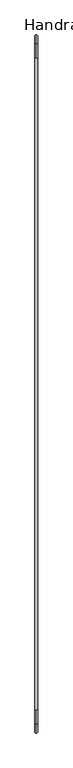
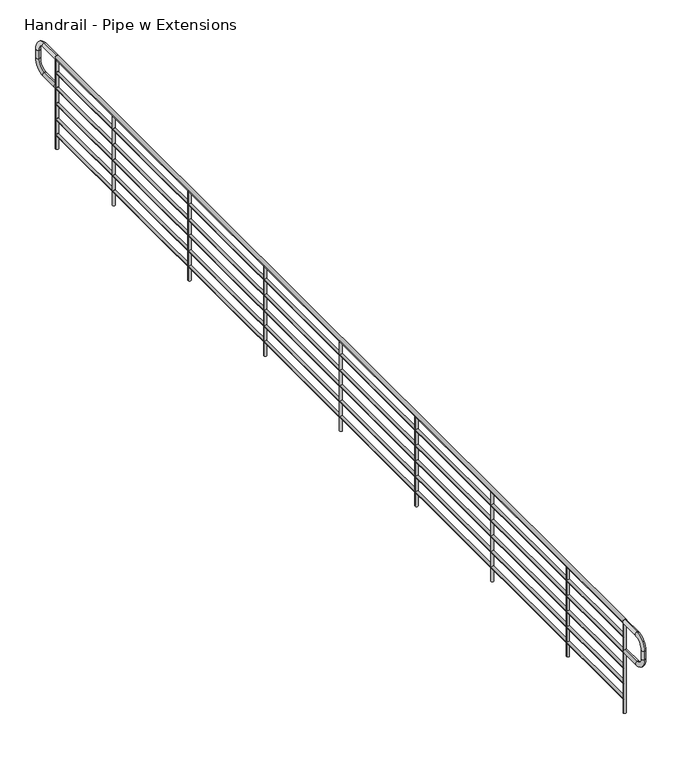
"""IFC4 building model written with IfcOpenShell, lengths in millimetres: railing geometry, Handrail - Pipe w Extensions."""

from ifc_helpers import new_model, si_unit, point, frame, frame_2d, origin, origin_with_axes, place, context, project, spatial, circle_curve, ellipse_curve, trimmed, segment, composite_curve, outline, extrude, source, transform, mapped, element, save
from ifc_brep_helpers import plane_surface, cylinder_surface, revolved_surface, advanced_brep


def handrail_pipe_w_extensions_4fdb8f92(model_context):
    return source(origin(), model_context, "Body", "SolidModel", [
        extrude(outline(composite_curve([segment(trimmed(circle_curve(frame_2d((895.35, -1497.5978678)), 19.05), [point((895.35, -1478.5478678))], [point((895.35, -1516.6478678))], False, "CARTESIAN"), True, "CONTINUOUS"), segment(trimmed(circle_curve(frame_2d((895.35, -1497.5978678)), 19.05), [point((895.35, -1516.6478678))], [point((895.35, -1478.5478678))], False, "CARTESIAN"), True, "CONTINUOUS")], self_intersect=False)), frame((0.0, -14489.4143828, 0.0), z_axis=(0.0, 1.0, 0.0), x_axis=(0.0, 0.0, 1.0)), (0.0, 0.0, 1.0), 9144.0),
        extrude(outline(composite_curve([segment(trimmed(circle_curve(frame_2d((749.3, -1497.5978678)), 12.7), [point((749.3, -1484.8978678))], [point((749.3, -1510.2978678))], False, "CARTESIAN"), True, "CONTINUOUS"), segment(trimmed(circle_curve(frame_2d((749.3, -1497.5978678)), 12.7), [point((749.3, -1510.2978678))], [point((749.3, -1484.8978678))], False, "CARTESIAN"), True, "CONTINUOUS")], self_intersect=False)), frame((0.0, -14489.4143828, 0.0), z_axis=(0.0, 1.0, 0.0), x_axis=(0.0, 0.0, 1.0)), (0.0, 0.0, 1.0), 9144.0),
        extrude(outline(composite_curve([segment(trimmed(circle_curve(frame_2d((596.9, -1497.5978678)), 12.7), [point((596.9, -1484.8978678))], [point((596.9, -1510.2978678))], False, "CARTESIAN"), True, "CONTINUOUS"), segment(trimmed(circle_curve(frame_2d((596.9, -1497.5978678)), 12.7), [point((596.9, -1510.2978678))], [point((596.9, -1484.8978678))], False, "CARTESIAN"), True, "CONTINUOUS")], self_intersect=False)), frame((0.0, -14489.4143828, 0.0), z_axis=(0.0, 1.0, 0.0), x_axis=(0.0, 0.0, 1.0)), (0.0, 0.0, 1.0), 9144.0),
        extrude(outline(composite_curve([segment(trimmed(circle_curve(frame_2d((444.5, -1497.5978678)), 12.7), [point((444.5, -1484.8978678))], [point((444.5, -1510.2978678))], False, "CARTESIAN"), True, "CONTINUOUS"), segment(trimmed(circle_curve(frame_2d((444.5, -1497.5978678)), 12.7), [point((444.5, -1510.2978678))], [point((444.5, -1484.8978678))], False, "CARTESIAN"), True, "CONTINUOUS")], self_intersect=False)), frame((0.0, -14489.4143828, 0.0), z_axis=(0.0, 1.0, 0.0), x_axis=(0.0, 0.0, 1.0)), (0.0, 0.0, 1.0), 9144.0),
        extrude(outline(composite_curve([segment(trimmed(circle_curve(frame_2d((292.1, -1497.5978678)), 12.7), [point((292.1, -1484.8978678))], [point((292.1, -1510.2978678))], False, "CARTESIAN"), True, "CONTINUOUS"), segment(trimmed(circle_curve(frame_2d((292.1, -1497.5978678)), 12.7), [point((292.1, -1510.2978678))], [point((292.1, -1484.8978678))], False, "CARTESIAN"), True, "CONTINUOUS")], self_intersect=False)), frame((0.0, -14489.4143828, 0.0), z_axis=(0.0, 1.0, 0.0), x_axis=(0.0, 0.0, 1.0)), (0.0, 0.0, 1.0), 9144.0),
        extrude(outline(composite_curve([segment(trimmed(circle_curve(frame_2d((139.7, -1497.5978678)), 12.7), [point((139.7, -1484.8978678))], [point((139.7, -1510.2978678))], False, "CARTESIAN"), True, "CONTINUOUS"), segment(trimmed(circle_curve(frame_2d((139.7, -1497.5978678)), 12.7), [point((139.7, -1510.2978678))], [point((139.7, -1484.8978678))], False, "CARTESIAN"), True, "CONTINUOUS")], self_intersect=False)), frame((0.0, -14489.4143828, 0.0), z_axis=(0.0, 1.0, 0.0), x_axis=(0.0, 0.0, 1.0)), (0.0, 0.0, 1.0), 9144.0),
        extrude(outline(composite_curve([segment(trimmed(circle_curve(frame_2d((-1497.5978678, -13575.0143828)), 12.7), [point((-1484.8978678, -13575.0143828))], [point((-1510.2978678, -13575.0143828))], False, "CARTESIAN"), True, "CONTINUOUS"), segment(trimmed(circle_curve(frame_2d((-1497.5978678, -13575.0143828)), 12.7), [point((-1510.2978678, -13575.0143828))], [point((-1484.8978678, -13575.0143828))], False, "CARTESIAN"), True, "CONTINUOUS")], self_intersect=False)), origin_with_axes(), (0.0, 0.0, 1.0), 876.3),
        extrude(outline(composite_curve([segment(trimmed(circle_curve(frame_2d((-1497.5978678, -12355.8143828)), 12.7), [point((-1484.8978678, -12355.8143828))], [point((-1510.2978678, -12355.8143828))], False, "CARTESIAN"), True, "CONTINUOUS"), segment(trimmed(circle_curve(frame_2d((-1497.5978678, -12355.8143828)), 12.7), [point((-1510.2978678, -12355.8143828))], [point((-1484.8978678, -12355.8143828))], False, "CARTESIAN"), True, "CONTINUOUS")], self_intersect=False)), origin_with_axes(), (0.0, 0.0, 1.0), 876.3),
        extrude(outline(composite_curve([segment(trimmed(circle_curve(frame_2d((-1497.5978678, -11136.6143828)), 12.7), [point((-1484.8978678, -11136.6143828))], [point((-1510.2978678, -11136.6143828))], False, "CARTESIAN"), True, "CONTINUOUS"), segment(trimmed(circle_curve(frame_2d((-1497.5978678, -11136.6143828)), 12.7), [point((-1510.2978678, -11136.6143828))], [point((-1484.8978678, -11136.6143828))], False, "CARTESIAN"), True, "CONTINUOUS")], self_intersect=False)), origin_with_axes(), (0.0, 0.0, 1.0), 876.3),
        extrude(outline(composite_curve([segment(trimmed(circle_curve(frame_2d((-1497.5978678, -9917.4143828)), 12.7), [point((-1484.8978678, -9917.4143828))], [point((-1510.2978678, -9917.4143828))], False, "CARTESIAN"), True, "CONTINUOUS"), segment(trimmed(circle_curve(frame_2d((-1497.5978678, -9917.4143828)), 12.7), [point((-1510.2978678, -9917.4143828))], [point((-1484.8978678, -9917.4143828))], False, "CARTESIAN"), True, "CONTINUOUS")], self_intersect=False)), origin_with_axes(), (0.0, 0.0, 1.0), 876.3),
        extrude(outline(composite_curve([segment(trimmed(circle_curve(frame_2d((-1497.5978678, -8698.2143828)), 12.7), [point((-1484.8978678, -8698.2143828))], [point((-1510.2978678, -8698.2143828))], False, "CARTESIAN"), True, "CONTINUOUS"), segment(trimmed(circle_curve(frame_2d((-1497.5978678, -8698.2143828)), 12.7), [point((-1510.2978678, -8698.2143828))], [point((-1484.8978678, -8698.2143828))], False, "CARTESIAN"), True, "CONTINUOUS")], self_intersect=False)), origin_with_axes(), (0.0, 0.0, 1.0), 876.3),
        extrude(outline(composite_curve([segment(trimmed(circle_curve(frame_2d((-1497.5978678, -7479.0143828)), 12.7), [point((-1484.8978678, -7479.0143828))], [point((-1510.2978678, -7479.0143828))], False, "CARTESIAN"), True, "CONTINUOUS"), segment(trimmed(circle_curve(frame_2d((-1497.5978678, -7479.0143828)), 12.7), [point((-1510.2978678, -7479.0143828))], [point((-1484.8978678, -7479.0143828))], False, "CARTESIAN"), True, "CONTINUOUS")], self_intersect=False)), origin_with_axes(), (0.0, 0.0, 1.0), 876.3),
        extrude(outline(composite_curve([segment(trimmed(circle_curve(frame_2d((-1497.5978678, -6259.8143828)), 12.7), [point((-1484.8978678, -6259.8143828))], [point((-1510.2978678, -6259.8143828))], False, "CARTESIAN"), True, "CONTINUOUS"), segment(trimmed(circle_curve(frame_2d((-1497.5978678, -6259.8143828)), 12.7), [point((-1510.2978678, -6259.8143828))], [point((-1484.8978678, -6259.8143828))], False, "CARTESIAN"), True, "CONTINUOUS")], self_intersect=False)), origin_with_axes(), (0.0, 0.0, 1.0), 876.3),
        advanced_brep(
        [(-1497.5978678, -14502.1143828, 628.65), (-1497.5978678, -14502.1143828, 590.55), (-1497.5978678, -14692.6143828, 628.65), (-1497.5978678, -14692.6143828, 590.55), (-1497.5978678, -14813.2643828, 711.2), (-1497.5978678, -14775.1643828, 711.2), (-1497.5978678, -14775.1643828, 793.75), (-1497.5978678, -14813.2643828, 793.75), (-1497.5978678, -14692.6143828, 914.4), (-1497.5978678, -14692.6143828, 876.3), (-1497.5978678, -14489.4143828, 876.3), (-1497.5978678, -14489.4143828, 914.4)],
        [
            (0, 1, circle_curve(frame((-1497.5978678, -14502.1143828, 609.6), z_axis=(0.0, 1.0, 0.0), x_axis=(0.0, 0.0, -1.0)), 19.05)),
            (1, 0, circle_curve(frame((-1497.5978678, -14502.1143828, 609.6), z_axis=(0.0, 1.0, 0.0), x_axis=(0.0, 0.0, -1.0)), 19.05)),
            (0, 2),
            (2, 3, circle_curve(frame((-1497.5978678, -14692.6143828, 609.6), z_axis=(0.0, 1.0, 0.0), x_axis=(0.0, 0.0, -1.0)), 19.05)),
            (3, 1),
            (3, 2, circle_curve(frame((-1497.5978678, -14692.6143828, 609.6), z_axis=(0.0, 1.0, 0.0), x_axis=(0.0, 0.0, -1.0)), 19.05)),
            (4, 3, circle_curve(frame((-1497.5978678, -14692.6143828, 711.2), z_axis=(1.0, 0.0, 0.0), x_axis=(0.0, 0.0, -1.0)), 120.65)),
            (2, 5, circle_curve(frame((-1497.5978678, -14692.6143828, 711.2), z_axis=(-1.0, 0.0, 0.0), x_axis=(0.0, 0.0, -1.0)), 82.55)),
            (5, 4, circle_curve(frame((-1497.5978678, -14794.2143828, 711.2), z_axis=(0.0, 0.0, -1.0), x_axis=(0.0, -1.0, 0.0)), 19.05)),
            (4, 5, circle_curve(frame((-1497.5978678, -14794.2143828, 711.2), z_axis=(0.0, 0.0, -1.0), x_axis=(0.0, -1.0, 0.0)), 19.05)),
            (5, 6),
            (6, 7, circle_curve(frame((-1497.5978678, -14794.2143828, 793.75), z_axis=(0.0, 0.0, -1.0), x_axis=(0.0, -1.0, 0.0)), 19.05)),
            (7, 4),
            (7, 6, circle_curve(frame((-1497.5978678, -14794.2143828, 793.75), z_axis=(0.0, 0.0, -1.0), x_axis=(0.0, -1.0, 0.0)), 19.05)),
            (8, 7, circle_curve(frame((-1497.5978678, -14692.6143828, 793.75), z_axis=(1.0, 0.0, 0.0), x_axis=(0.0, -1.0, 0.0)), 120.65)),
            (6, 9, circle_curve(frame((-1497.5978678, -14692.6143828, 793.75), z_axis=(-1.0, 0.0, 0.0), x_axis=(0.0, -1.0, 0.0)), 82.55)),
            (9, 8, circle_curve(frame((-1497.5978678, -14692.6143828, 895.35), z_axis=(0.0, -1.0, 0.0), x_axis=(0.0, 0.0, 1.0)), 19.05)),
            (8, 9, circle_curve(frame((-1497.5978678, -14692.6143828, 895.35), z_axis=(0.0, -1.0, 0.0), x_axis=(0.0, 0.0, 1.0)), 19.05)),
            (10, 11, circle_curve(frame((-1497.5978678, -14489.4143828, 895.35), z_axis=(0.0, 1.0, 0.0), x_axis=(0.0, 0.0, 1.0)), 19.05)),
            (11, 10, circle_curve(frame((-1497.5978678, -14489.4143828, 895.35), z_axis=(0.0, 1.0, 0.0), x_axis=(0.0, 0.0, 1.0)), 19.05)),
            (9, 10),
            (11, 8),
        ],
        [
            plane_surface(frame((-1516.6478678, -14502.1143828, 609.6), z_axis=(0.0, 1.0, 0.0), x_axis=(0.0, 0.0, -1.0))),
            cylinder_surface(frame((-1497.5978678, -14502.1143828, 609.6), z_axis=(0.0, 1.0, 0.0), x_axis=(0.0, 0.0, -1.0)), 19.05),
            revolved_surface(trimmed(ellipse_curve(frame((-1497.5978678, -14692.6143828, 609.6), z_axis=(0.0, 1.0, 0.0), x_axis=(0.0, 0.0, -1.0)), 19.05, 19.05), [point((-1497.5978678, -14692.6143828, 628.65))], [point((-1497.5978678, -14692.6143828, 590.55))], True, "CARTESIAN"), (-1497.5978678, -14692.6143828, 711.2), (-1.0, 0.0, 0.0)),
            revolved_surface(trimmed(ellipse_curve(frame((-1497.5978678, -14692.6143828, 609.6), z_axis=(0.0, 1.0, 0.0), x_axis=(0.0, 0.0, -1.0)), 19.05, 19.05), [point((-1497.5978678, -14692.6143828, 590.55))], [point((-1497.5978678, -14692.6143828, 628.65))], True, "CARTESIAN"), (-1497.5978678, -14692.6143828, 711.2), (-1.0, 0.0, 0.0)),
            cylinder_surface(frame((-1497.5978678, -14794.2143828, 711.2), z_axis=(0.0, 0.0, -1.0), x_axis=(0.0, -1.0, 0.0)), 19.05),
            revolved_surface(trimmed(ellipse_curve(frame((-1497.5978678, -14794.2143828, 793.75), z_axis=(0.0, 0.0, -1.0), x_axis=(0.0, -1.0, 0.0)), 19.05, 19.05), [point((-1497.5978678, -14775.1643828, 793.75))], [point((-1497.5978678, -14813.2643828, 793.75))], True, "CARTESIAN"), (-1497.5978678, -14692.6143828, 793.75), (-1.0, 0.0, 0.0)),
            revolved_surface(trimmed(ellipse_curve(frame((-1497.5978678, -14794.2143828, 793.75), z_axis=(0.0, 0.0, -1.0), x_axis=(0.0, -1.0, 0.0)), 19.05, 19.05), [point((-1497.5978678, -14813.2643828, 793.75))], [point((-1497.5978678, -14775.1643828, 793.75))], True, "CARTESIAN"), (-1497.5978678, -14692.6143828, 793.75), (-1.0, 0.0, 0.0)),
            plane_surface(frame((-1516.6478678, -14489.4143828, 895.35), z_axis=(0.0, 1.0, 0.0), x_axis=(0.0, 0.0, 1.0))),
            cylinder_surface(frame((-1497.5978678, -14692.6143828, 895.35), z_axis=(0.0, -1.0, 0.0), x_axis=(0.0, 0.0, 1.0)), 19.05),
        ],
        [
            (0, [[1, 2]]),
            (1, [[-1, 3, 4, 5]]),
            (1, [[-2, -5, 6, -3]]),
            (2, [[7, -4, 8, 9]]),
            (3, [[-8, -6, -7, 10]]),
            (4, [[-9, 11, 12, 13]]),
            (4, [[-10, -13, 14, -11]]),
            (5, [[15, -12, 16, 17]]),
            (6, [[-16, -14, -15, 18]]),
            (7, [[19, 20]]),
            (8, [[-17, 21, -20, 22]]),
            (8, [[-18, -22, -19, -21]]),
        ],
    ),
        extrude(outline(composite_curve([segment(trimmed(circle_curve(frame_2d((-1497.5978678, -14489.4143828)), 12.7), [point((-1510.2978678, -14489.4143828))], [point((-1484.8978678, -14489.4143828))], False, "CARTESIAN"), True, "CONTINUOUS"), segment(trimmed(circle_curve(frame_2d((-1497.5978678, -14489.4143828)), 12.7), [point((-1484.8978678, -14489.4143828))], [point((-1510.2978678, -14489.4143828))], False, "CARTESIAN"), True, "CONTINUOUS")], self_intersect=False)), origin_with_axes(), (0.0, 0.0, 1.0), 876.3),
        advanced_brep(
        [(-1497.5978678, -5345.4143828, 876.3), (-1497.5978678, -5345.4143828, 914.4), (-1497.5978678, -5142.2143828, 876.3), (-1497.5978678, -5142.2143828, 914.4), (-1497.5978678, -5021.5643828, 793.75), (-1497.5978678, -5059.6643828, 793.75), (-1497.5978678, -5059.6643828, 711.2), (-1497.5978678, -5021.5643828, 711.2), (-1497.5978678, -5142.2143828, 590.55), (-1497.5978678, -5142.2143828, 628.65), (-1497.5978678, -5332.7143828, 628.65), (-1497.5978678, -5332.7143828, 590.55)],
        [
            (0, 1, circle_curve(frame((-1497.5978678, -5345.4143828, 895.35), z_axis=(0.0, -1.0, 0.0), x_axis=(0.0, 0.0, 1.0)), 19.05)),
            (1, 0, circle_curve(frame((-1497.5978678, -5345.4143828, 895.35), z_axis=(0.0, -1.0, 0.0), x_axis=(0.0, 0.0, 1.0)), 19.05)),
            (0, 2),
            (2, 3, circle_curve(frame((-1497.5978678, -5142.2143828, 895.35), z_axis=(0.0, -1.0, 0.0), x_axis=(0.0, 0.0, 1.0)), 19.05)),
            (3, 1),
            (3, 2, circle_curve(frame((-1497.5978678, -5142.2143828, 895.35), z_axis=(0.0, -1.0, 0.0), x_axis=(0.0, 0.0, 1.0)), 19.05)),
            (4, 3, circle_curve(frame((-1497.5978678, -5142.2143828, 793.75), z_axis=(1.0, 0.0, 0.0), x_axis=(0.0, 0.0, 1.0)), 120.65)),
            (2, 5, circle_curve(frame((-1497.5978678, -5142.2143828, 793.75), z_axis=(-1.0, 0.0, 0.0), x_axis=(0.0, 0.0, 1.0)), 82.55)),
            (5, 4, circle_curve(frame((-1497.5978678, -5040.6143828, 793.75), z_axis=(0.0, 0.0, 1.0), x_axis=(0.0, 1.0, 0.0)), 19.05)),
            (4, 5, circle_curve(frame((-1497.5978678, -5040.6143828, 793.75), z_axis=(0.0, 0.0, 1.0), x_axis=(0.0, 1.0, 0.0)), 19.05)),
            (5, 6),
            (6, 7, circle_curve(frame((-1497.5978678, -5040.6143828, 711.2), z_axis=(0.0, 0.0, 1.0), x_axis=(0.0, 1.0, 0.0)), 19.05)),
            (7, 4),
            (7, 6, circle_curve(frame((-1497.5978678, -5040.6143828, 711.2), z_axis=(0.0, 0.0, 1.0), x_axis=(0.0, 1.0, 0.0)), 19.05)),
            (8, 7, circle_curve(frame((-1497.5978678, -5142.2143828, 711.2), z_axis=(1.0, 0.0, 0.0), x_axis=(0.0, 1.0, 0.0)), 120.65)),
            (6, 9, circle_curve(frame((-1497.5978678, -5142.2143828, 711.2), z_axis=(-1.0, 0.0, 0.0), x_axis=(0.0, 1.0, 0.0)), 82.55)),
            (9, 8, circle_curve(frame((-1497.5978678, -5142.2143828, 609.6), z_axis=(0.0, 1.0, 0.0), x_axis=(0.0, 0.0, -1.0)), 19.05)),
            (8, 9, circle_curve(frame((-1497.5978678, -5142.2143828, 609.6), z_axis=(0.0, 1.0, 0.0), x_axis=(0.0, 0.0, -1.0)), 19.05)),
            (10, 11, circle_curve(frame((-1497.5978678, -5332.7143828, 609.6), z_axis=(0.0, -1.0, 0.0), x_axis=(0.0, 0.0, -1.0)), 19.05)),
            (11, 10, circle_curve(frame((-1497.5978678, -5332.7143828, 609.6), z_axis=(0.0, -1.0, 0.0), x_axis=(0.0, 0.0, -1.0)), 19.05)),
            (9, 10),
            (11, 8),
        ],
        [
            plane_surface(frame((-1516.6478678, -5345.4143828, 895.35), z_axis=(0.0, -1.0, 0.0), x_axis=(0.0, 0.0, 1.0))),
            cylinder_surface(frame((-1497.5978678, -5345.4143828, 895.35), z_axis=(0.0, -1.0, 0.0), x_axis=(0.0, 0.0, 1.0)), 19.05),
            revolved_surface(trimmed(ellipse_curve(frame((-1497.5978678, -5142.2143828, 895.35), z_axis=(0.0, -1.0, 0.0), x_axis=(0.0, 0.0, 1.0)), 19.05, 19.05), [point((-1497.5978678, -5142.2143828, 876.3))], [point((-1497.5978678, -5142.2143828, 914.4))], True, "CARTESIAN"), (-1497.5978678, -5142.2143828, 793.75), (-1.0, 0.0, 0.0)),
            revolved_surface(trimmed(ellipse_curve(frame((-1497.5978678, -5142.2143828, 895.35), z_axis=(0.0, -1.0, 0.0), x_axis=(0.0, 0.0, 1.0)), 19.05, 19.05), [point((-1497.5978678, -5142.2143828, 914.4))], [point((-1497.5978678, -5142.2143828, 876.3))], True, "CARTESIAN"), (-1497.5978678, -5142.2143828, 793.75), (-1.0, 0.0, 0.0)),
            cylinder_surface(frame((-1497.5978678, -5040.6143828, 793.75), z_axis=(0.0, 0.0, 1.0), x_axis=(0.0, 1.0, 0.0)), 19.05),
            revolved_surface(trimmed(ellipse_curve(frame((-1497.5978678, -5040.6143828, 711.2), z_axis=(0.0, 0.0, 1.0), x_axis=(0.0, 1.0, 0.0)), 19.05, 19.05), [point((-1497.5978678, -5059.6643828, 711.2))], [point((-1497.5978678, -5021.5643828, 711.2))], True, "CARTESIAN"), (-1497.5978678, -5142.2143828, 711.2), (-1.0, 0.0, 0.0)),
            revolved_surface(trimmed(ellipse_curve(frame((-1497.5978678, -5040.6143828, 711.2), z_axis=(0.0, 0.0, 1.0), x_axis=(0.0, 1.0, 0.0)), 19.05, 19.05), [point((-1497.5978678, -5021.5643828, 711.2))], [point((-1497.5978678, -5059.6643828, 711.2))], True, "CARTESIAN"), (-1497.5978678, -5142.2143828, 711.2), (-1.0, 0.0, 0.0)),
            plane_surface(frame((-1516.6478678, -5332.7143828, 609.6), z_axis=(0.0, -1.0, 0.0), x_axis=(0.0, 0.0, -1.0))),
            cylinder_surface(frame((-1497.5978678, -5142.2143828, 609.6), z_axis=(0.0, 1.0, 0.0), x_axis=(0.0, 0.0, -1.0)), 19.05),
        ],
        [
            (0, [[1, 2]]),
            (1, [[-1, 3, 4, 5]]),
            (1, [[-2, -5, 6, -3]]),
            (2, [[7, -4, 8, 9]]),
            (3, [[-8, -6, -7, 10]]),
            (4, [[-9, 11, 12, 13]]),
            (4, [[-10, -13, 14, -11]]),
            (5, [[15, -12, 16, 17]]),
            (6, [[-16, -14, -15, 18]]),
            (7, [[19, 20]]),
            (8, [[-17, 21, -20, 22]]),
            (8, [[-18, -22, -19, -21]]),
        ],
    ),
        extrude(outline(composite_curve([segment(trimmed(circle_curve(frame_2d((-1497.5978678, -5345.4143828)), 12.7), [point((-1510.2978678, -5345.4143828))], [point((-1484.8978678, -5345.4143828))], False, "CARTESIAN"), True, "CONTINUOUS"), segment(trimmed(circle_curve(frame_2d((-1497.5978678, -5345.4143828)), 12.7), [point((-1484.8978678, -5345.4143828))], [point((-1510.2978678, -5345.4143828))], False, "CARTESIAN"), True, "CONTINUOUS")], self_intersect=False)), origin_with_axes(), (0.0, 0.0, 1.0), 876.3),
    ])


if __name__ == "__main__":
    model = new_model("IFC4")
    model_context = context("Model", 3, world=origin())
    ifc_project = project(units=[si_unit("LENGTHUNIT", "METRE", prefix="MILLI")], contexts=[model_context])
    site = spatial("IfcSite", under=ifc_project)
    building = spatial("IfcBuilding", under=site)
    placement = place(None, origin())
    handrail_pipe_w_extensions_shape = handrail_pipe_w_extensions_4fdb8f92(model_context)
    element("IfcRailing", 1, ObjectType="Handrail - Pipe w Extensions", at=placement, inside=building, context=model_context, shape_type="MappedRepresentation", body=[
        mapped(handrail_pipe_w_extensions_shape, transform((0.0, 0.0, 0.0), x_axis=(1.0, 0.0, 0.0), y_axis=(0.0, 1.0, 0.0), z_axis=(0.0, 0.0, 1.0))),
    ])
    save(model, "model.ifc")
